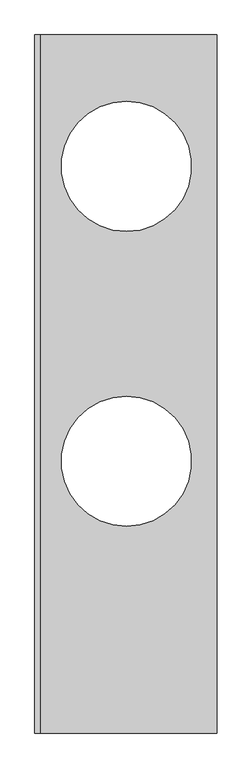
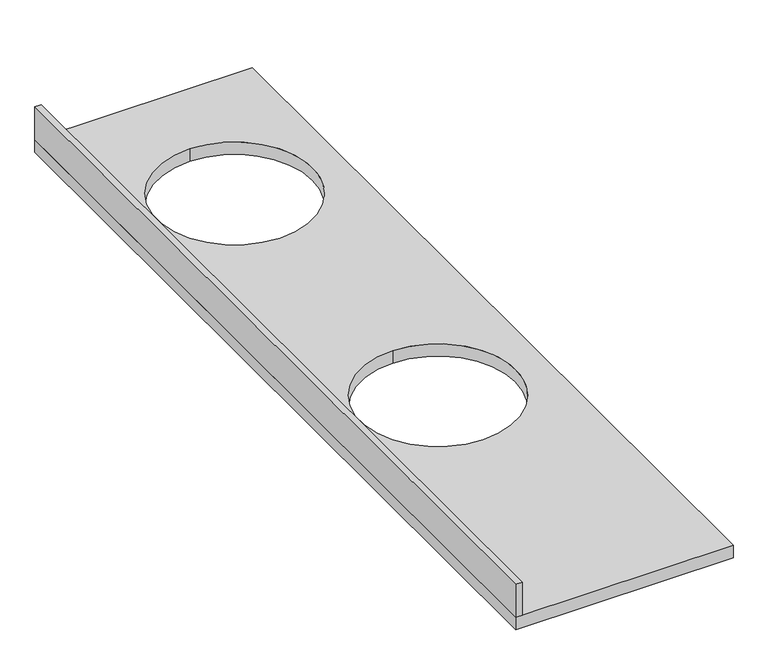
"""IFC4 building model written with IfcOpenShell, lengths in millimetres: furniture geometry."""

from ifc_helpers import new_model, si_unit, point, frame, frame_2d, origin, place, context, project, spatial, polyline, circle_curve, trimmed, segment, composite_curve, outline, extrude, source, transform, mapped, element, save


def furniture_a217bf1b(model_context):
    return source(origin(), model_context, "Body", "SweptSolid", [
        extrude(outline(polyline([(648262.3617239, -569560.2257591), (648262.3617239, -571990.2913841), (648243.3117239, -571990.2913841), (648243.3117239, -569560.2257591), (648262.3617239, -569560.2257591)])), frame((0.0, 0.0, 787.4), z_axis=(0.0, 0.0, 1.0), x_axis=(1.0, 0.0, 0.0)), (0.0, 0.0, 1.0), 101.6),
        extrude(outline(polyline([(648878.3117239, -571990.2913841), (648243.3117239, -571990.2913841), (648243.3117239, -569560.2257591), (648878.3117239, -569560.2257591), (648878.3117239, -571990.2913841)]), holes=[composite_curve([segment(trimmed(circle_curve(frame_2d((648562.5970089, -571044.1413841)), 226.814715), [point((648562.5970089, -571270.9560991))], [point((648562.5970089, -570817.3266691))], True, "CARTESIAN"), True, "CONTINUOUS"), segment(trimmed(circle_curve(frame_2d((648562.5970089, -571044.1413841)), 226.814715), [point((648562.5970089, -570817.3266691))], [point((648562.5970089, -571270.9560991))], True, "CARTESIAN"), True, "CONTINUOUS")], self_intersect=False), composite_curve([segment(trimmed(circle_curve(frame_2d((648562.5970089, -570017.4257591)), 226.814715), [point((648562.5970089, -570244.2404741))], [point((648562.5970089, -569790.6110441))], True, "CARTESIAN"), True, "CONTINUOUS"), segment(trimmed(circle_curve(frame_2d((648562.5970089, -570017.4257591)), 226.814715), [point((648562.5970089, -569790.6110441))], [point((648562.5970089, -570244.2404741))], True, "CARTESIAN"), True, "CONTINUOUS")], self_intersect=False)]), frame((0.0, 0.0, 749.3), z_axis=(0.0, 0.0, 1.0), x_axis=(1.0, 0.0, 0.0)), (0.0, 0.0, 1.0), 38.1),
    ])


if __name__ == "__main__":
    model = new_model("IFC4")
    model_context = context("Model", 3, world=origin())
    ifc_project = project(units=[si_unit("LENGTHUNIT", "METRE", prefix="MILLI")], contexts=[model_context])
    site = spatial("IfcSite", under=ifc_project)
    building = spatial("IfcBuilding", under=site)
    placement = place(None, origin())
    furniture_shape = furniture_a217bf1b(model_context)
    element("IfcFurniture", 1, ObjectType="Vanity Counter Top w 2 Round Sink Holes:72\":2372:72\":2372 : Vanity Counter Top w 2 Round Sink Holes:72\":2372:300229 : Vanity Counter Top w 2 Round Sink Holes:72\":2372:72\":2372 : Vanity Counter Top w 2 Round Sink Holes:72\":2372:300229", at=placement, inside=building, context=model_context, shape_type="MappedRepresentation", body=[
        mapped(furniture_shape, transform((0.0, 0.0, 0.0), x_axis=(1.0, 0.0, 0.0), y_axis=(0.0, 1.0, 0.0), z_axis=(0.0, 0.0, 1.0))),
    ])
    save(model, "model.ifc")

# Revit data of these elements
# Type "Vanity Counter Top w 2 Round Sink Holes:72\":2372:72\":2372 : Vanity Counter Top w 2 Round Sink Holes:72\":2372:300229 : Vanity Counter Top w 2 Round Sink Holes:72\":2372:72\":2372 : Vanity Counter Top w 2 Round Sink Holes:72\":2372:300229"
#   NameOverride = "Vanity Counter Top w 2 Round Sink Holes:72\":2372:72\":2372 : Vanity Counter Top w 2 Round Sink Holes:72\":2372:300229"
#   ObjectTypeOverride = "72\":2372 : Vanity Counter Top w 2 Round Sink Holes:72\":2372"
#   Tag = "300229"
# Element 1 (IfcFurniture, "Vanity Counter Top w 2 Round Sink Holes:72\":2372:72\":2372 : Vanity Counter Top w 2 Round Sink Holes:72\":2372:300229 : Vanity Counter Top w 2 Round Sink Holes:72\":2372:72\":2372 : Vanity Counter Top w 2 Round Sink Holes:72\":2372:300229")
#   Materials on its faces: "Counter Top"
# Materials
#   "Counter Top": class "Unassigned", colour RGB 226 177 128, transparency 0
